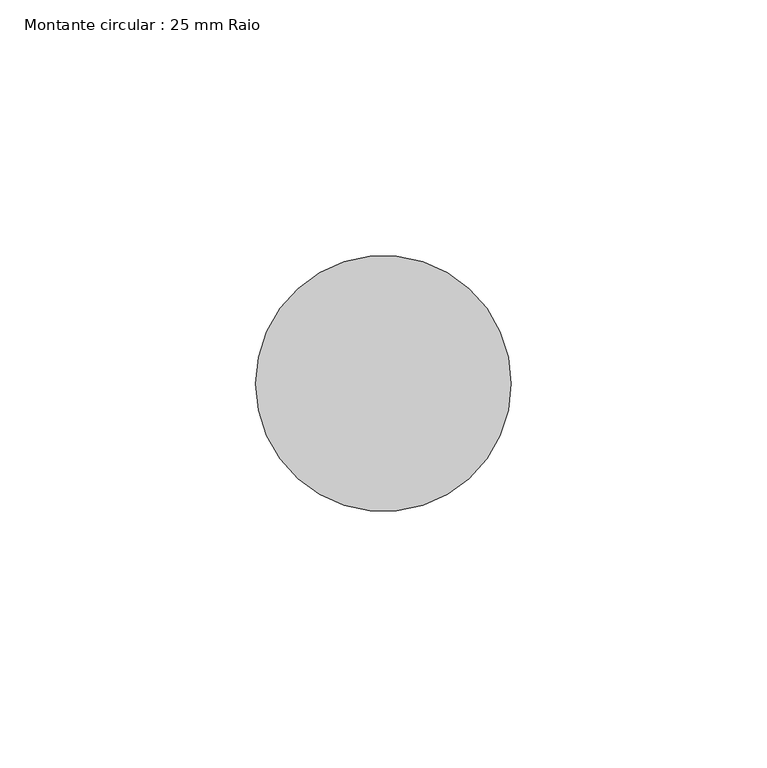
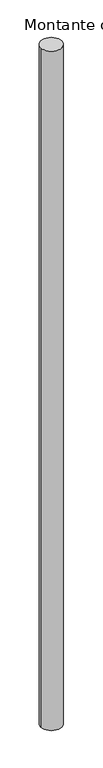
"""IFC4 building model written with IfcOpenShell, lengths in millimetres: member geometry, Montante circular : 25 mm Raio."""

from ifc_helpers import new_model, si_unit, point, frame, frame_2d, origin, place, context, project, spatial, circle_curve, trimmed, segment, composite_curve, outline, extrude, source, transform, mapped, element, save


def montante_circular_25_mm_raio_e9b0e8a5(model_context):
    return source(origin(), model_context, "Body", "SweptSolid", [
        extrude(outline(composite_curve([segment(trimmed(circle_curve(frame_2d((-25.0, 0.0)), 25.0), [point((0.0, 0.0))], [point((-50.0, 0.0))], False, "CARTESIAN"), True, "CONTINUOUS"), segment(trimmed(circle_curve(frame_2d((-25.0, 0.0)), 25.0), [point((-50.0, 0.0))], [point((0.0, 0.0))], False, "CARTESIAN"), True, "CONTINUOUS")], self_intersect=False)), frame((0.0, 0.0, -1716.7125085), z_axis=(0.0, 0.0, 1.0), x_axis=(1.0, 0.0, 0.0)), (0.0, 0.0, 1.0), 1716.7125085),
    ])


if __name__ == "__main__":
    model = new_model("IFC4")
    model_context = context("Model", 3, world=origin())
    ifc_project = project(units=[si_unit("LENGTHUNIT", "METRE", prefix="MILLI")], contexts=[model_context])
    site = spatial("IfcSite", under=ifc_project)
    building = spatial("IfcBuilding", under=site)
    placement = place(None, origin())
    montante_circular_25_mm_raio_shape = montante_circular_25_mm_raio_e9b0e8a5(model_context)
    element("IfcMember", 1, ObjectType="Montante circular : 25 mm Raio", at=placement, inside=building, context=model_context, shape_type="MappedRepresentation", body=[
        mapped(montante_circular_25_mm_raio_shape, transform((0.0, 0.0, 0.0), x_axis=(1.0, 0.0, 0.0), y_axis=(0.0, 1.0, 0.0), z_axis=(0.0, 0.0, 1.0))),
    ])
    save(model, "model.ifc")

# Revit data of these elements
# Type "Montante circular : 25 mm Raio"
#   built-in parameter 1007350 = 0.082021 (stored number, unit not read)
# Element 1 (IfcMember, "Montante circular : 25 mm Raio")
#   Materials on its faces: "Alumín."
# Materials
#   "Alumín.": class "Metal", colour RGB 247 247 247, transparency 0, Description = "Alumín. 6061", Cost = 0
